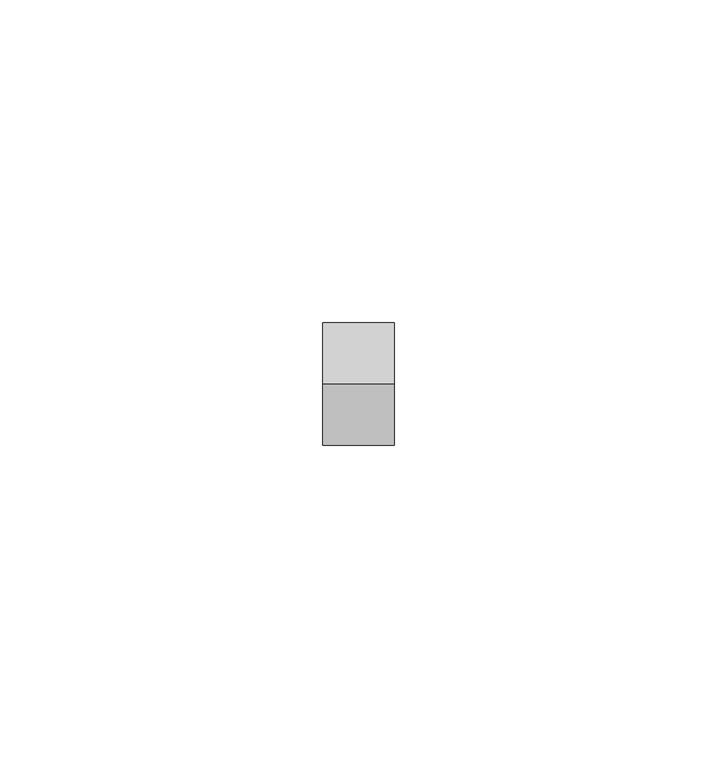
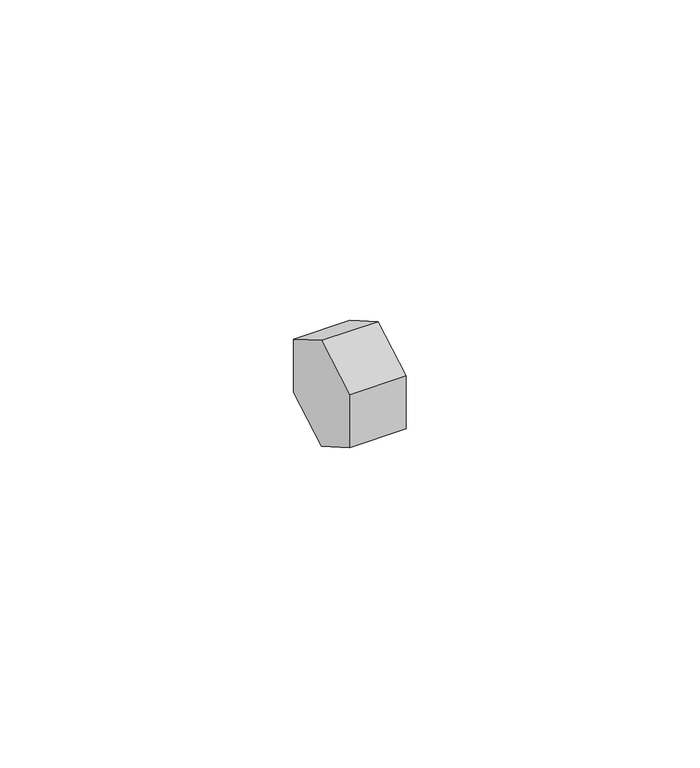
"""IFC4 building model written with IfcOpenShell, lengths in millimetres: proxy geometry, Generic Models 7:Generic Models 1:8:Generic Models 1:8 : Generic Models 7:Generic Models 1:337419:59 : Generic Models 7:Generic Models 1:8:Generic Models 1:8 : Generic Models 7:Generic Models 1:337419:315935."""

from ifc_helpers import new_model, si_unit, frame, origin, place, context, project, spatial, polyline, outline, extrude, source, transform, mapped, element, save


def generic_models_eda03d1c(model_context):
    return source(origin(), model_context, "Body", "SweptSolid", [
        extrude(outline(polyline([(-564915.9326015, 8757.3782009), (-564925.4576015, 8762.8774622), (-564925.4576015, 8773.8759848), (-564915.9326015, 8779.3752461), (-564906.4076015, 8773.8759848), (-564906.4076015, 8762.8774622), (-564915.9326015, 8757.3782009)])), frame((593654.1476618, 0.0, 0.0), z_axis=(1.0, 0.0, 0.0), x_axis=(0.0, 1.0, 0.0)), (0.0, 0.0, 1.0), 11.1125),
    ])


if __name__ == "__main__":
    model = new_model("IFC4")
    model_context = context("Model", 3, world=origin())
    ifc_project = project(units=[si_unit("LENGTHUNIT", "METRE", prefix="MILLI")], contexts=[model_context])
    site = spatial("IfcSite", under=ifc_project)
    building = spatial("IfcBuilding", under=site)
    placement = place(None, origin())
    generic_models_shape = generic_models_eda03d1c(model_context)
    element("IfcBuildingElementProxy", 1, Name="Generic Models 7:Generic Models 1:8:Generic Models 1:8 : Generic Models 7:Generic Models 1:337419:59 : Generic Models 7:Generic Models 1:8:Generic Models 1:8 : Generic Models 7:Generic Models 1:337419:315935", ObjectType="Generic Models 7:Generic Models 1:8:Generic Models 1:8 : Generic Models 7:Generic Models 1:337419:59 : Generic Models 7:Generic Models 1:8:Generic Models 1:8 : Generic Models 7:Generic Models 1:337419:315935", at=placement, inside=building, context=model_context, shape_type="MappedRepresentation", body=[
        mapped(generic_models_shape, transform((0.0, 0.0, 0.0), x_axis=(1.0, 0.0, 0.0), y_axis=(0.0, 1.0, 0.0), z_axis=(0.0, 0.0, 1.0))),
    ])
    save(model, "model.ifc")

# Revit data of these elements
# Type "Generic Models 7:Generic Models 1:8:Generic Models 1:8 : Generic Models 7:Generic Models 1:337419:59 : Generic Models 7:Generic Models 1:8:Generic Models 1:8 : Generic Models 7:Generic Models 1:337419:315935"
#   NameOverride = "Generic Models 7:Generic Models 1:8:Generic Models 1:8 : Generic Models 7:Generic Models 1:337419:315935"
#   ObjectTypeOverride = "Generic Models 1:8 : Generic Models 7:Generic Models 1:337419"
#   Reference = "Generic Models 1"
#   Tag = "315935"
# Element 1 (IfcBuildingElementProxy, "Generic Models 7:Generic Models 1:8:Generic Models 1:8 : Generic Models 7:Generic Models 1:337419:59 : Generic Models 7:Generic Models 1:8:Generic Models 1:8 : Generic Models 7:Generic Models 1:337419:315935")
#   Materials on its faces: "1/2\" THRU BOLTS"
# Materials
#   "1/2\" THRU BOLTS": class "Generic", colour RGB 120 120 120, transparency 0, Cost = 0
